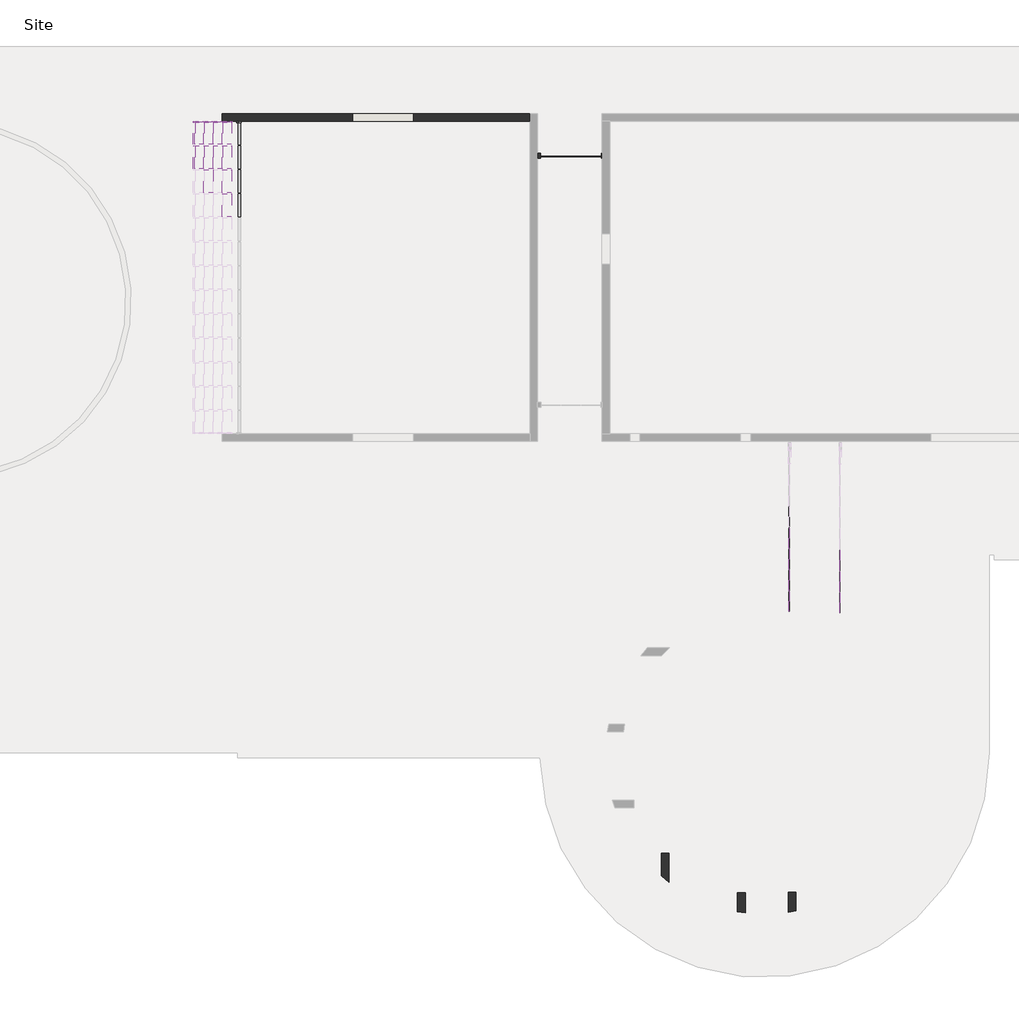
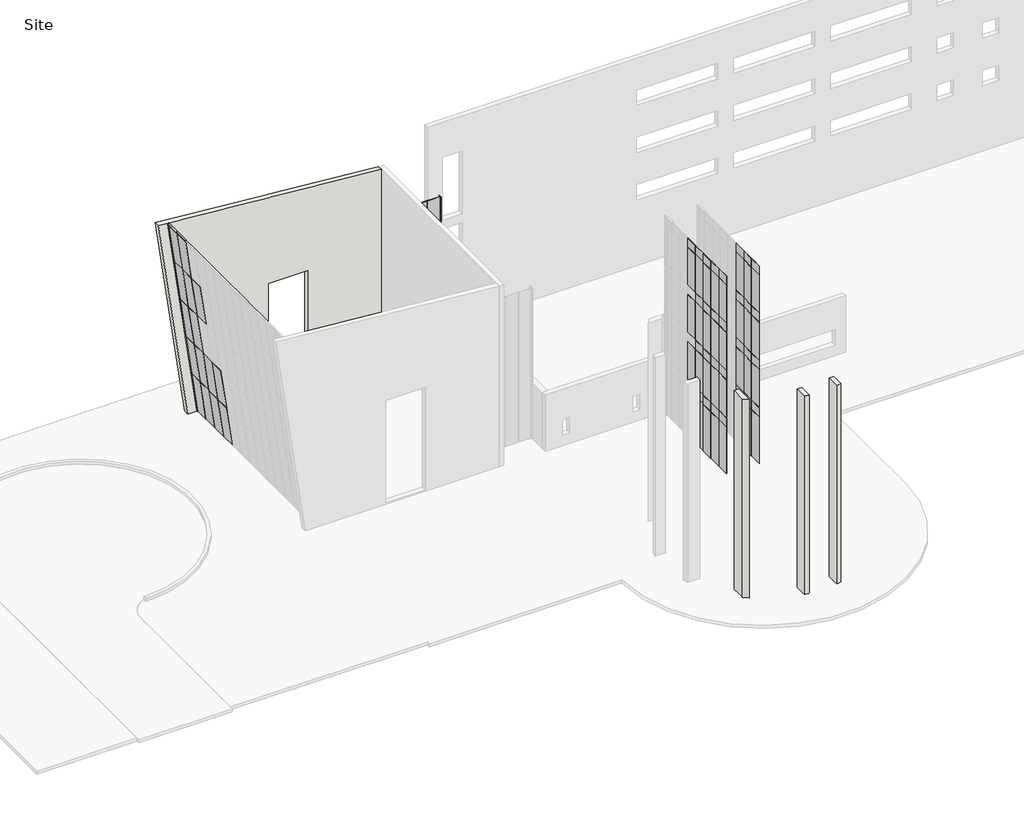
# One storey, part 2 of 4: 79 plates, 7 members, 6 walls.
"""IFC4 building model written with IfcOpenShell, lengths in millimetres."""

import ifcopenshell
import ifcopenshell.guid

model = None  # the IFC model being written
_history = None  # IfcOwnerHistory: only IFC2X3 demands one
_inside = {}  # id of a spatial element -> (the spatial element, [elements in it])
_under = {}  # id of a project, library or spatial element -> (it, [spatial elements below it])
_declared = {}  # id of a project -> (the project, [libraries it declares])
_typed = {}  # id of a type object -> (the type object, [elements of that type])
_made_of = {}  # id of a material, layer set ... -> (it, [elements and type objects made of it])


def new_model(schema):
    """Start an empty IFC model of exactly this schema.

    Asked for "IFC4X3", IfcOpenShell would pick the latest addendum, in which some entities
    have other attributes; the version numbers below select the first issue.
    IFC2X3 requires an IfcOwnerHistory on every rooted entity: one is made here for all.
    """
    global model, _history
    if schema == "IFC4X3":
        model = ifcopenshell.file(schema_version=(4, 3, 0, 0))
    else:
        model = ifcopenshell.file(schema=schema)
    _inside.clear()
    _under.clear()
    _declared.clear()
    _typed.clear()
    _made_of.clear()
    _history = None
    if model.schema == "IFC2X3":
        org = make("IfcOrganization", Name="unknown")
        user = make(
            "IfcPersonAndOrganization",
            ThePerson=make("IfcPerson", FamilyName="unknown"),
            TheOrganization=org,
        )
        app = make(
            "IfcApplication",
            ApplicationDeveloper=org,
            Version="unknown",
            ApplicationFullName="unknown",
            ApplicationIdentifier="unknown",
        )
        _history = make(
            "IfcOwnerHistory",
            OwningUser=user,
            OwningApplication=app,
            ChangeAction="ADDED",
            CreationDate=0,
        )
    return model


def make(cls, **values):
    """One entity of the class cls with the attributes given. An attribute that is None is left unset."""
    return model.create_entity(
        cls, **{name: value for name, value in values.items() if value is not None}
    )


def rooted(cls, **values):
    """An entity with a GlobalId (a new one), such as an element, a storey or a relation."""
    return make(cls, GlobalId=ifcopenshell.guid.new(), OwnerHistory=_history, **values)


def si_unit(unit_type, name, prefix=None):
    """IfcSIUnit, for example si_unit("LENGTHUNIT", "METRE", prefix="MILLI")."""
    return make("IfcSIUnit", UnitType=unit_type, Prefix=prefix, Name=name)


def assignment(units):
    """IfcUnitAssignment: the units of a project."""
    return None if units is None else make("IfcUnitAssignment", Units=units)


def point(xyz):
    """IfcCartesianPoint."""
    return None if xyz is None else make("IfcCartesianPoint", Coordinates=xyz)


def direction(xyz):
    """IfcDirection."""
    return None if xyz is None else make("IfcDirection", DirectionRatios=xyz)


def frame(location, z_axis=None, x_axis=None):
    """IfcAxis2Placement3D, a coordinate frame: its origin and axes. An axis left out is left unset."""
    return make(
        "IfcAxis2Placement3D",
        Location=point(location),
        Axis=direction(z_axis),
        RefDirection=direction(x_axis),
    )


def frame_2d(location, x_axis=None):
    """IfcAxis2Placement2D, a coordinate frame in the plane: its origin and x axis."""
    return make(
        "IfcAxis2Placement2D", Location=point(location), RefDirection=direction(x_axis)
    )


def origin():
    """The frame at (0, 0, 0) with its axes left unset."""
    return frame((0.0, 0.0, 0.0))


def origin_with_axes():
    """The frame at (0, 0, 0) with the z axis (0, 0, 1) and the x axis (1, 0, 0) written out."""
    return frame((0.0, 0.0, 0.0), z_axis=(0.0, 0.0, 1.0), x_axis=(1.0, 0.0, 0.0))


def place(relative_to, where):
    """IfcLocalPlacement: puts the frame where relative to a parent placement (None: the world)."""
    return make(
        "IfcLocalPlacement", PlacementRelTo=relative_to, RelativePlacement=where
    )


def context(
    kind, dimensions, precision=None, world=None, true_north=None, identifier=None
):
    """IfcGeometricRepresentationContext, for example the 3D "Model" context."""
    return make(
        "IfcGeometricRepresentationContext",
        ContextIdentifier=identifier,
        ContextType=kind,
        CoordinateSpaceDimension=dimensions,
        Precision=precision,
        WorldCoordinateSystem=world,
        TrueNorth=true_north,
    )


def project(units=None, contexts=None):
    """IfcProject with its units and contexts."""
    return rooted(
        "IfcProject",
        Name="project",
        RepresentationContexts=contexts,
        UnitsInContext=assignment(units),
    )


def spatial(cls, under=None, at=None, **own):
    """A site, building, storey or space (cls), placed at a placement, below another one or the project."""
    s = rooted(cls, ObjectPlacement=at, **own)
    if under is not None:
        _under.setdefault(under.id(), (under, []))[1].append(s)
    return s


def polyline(points):
    """IfcPolyline through the points."""
    return make("IfcPolyline", Points=[point(p) for p in points])


def circle_curve(where, radius):
    """IfcCircle in the frame where."""
    return make("IfcCircle", Position=where, Radius=radius)


def trimmed(basis, trim1, trim2, sense, master):
    """IfcTrimmedCurve: the piece of a basis curve between two trims."""
    return make(
        "IfcTrimmedCurve",
        BasisCurve=basis,
        Trim1=trim1,
        Trim2=trim2,
        SenseAgreement=sense,
        MasterRepresentation=master,
    )


def segment(curve, same_sense, transition):
    """IfcCompositeCurveSegment."""
    return make(
        "IfcCompositeCurveSegment",
        Transition=transition,
        SameSense=same_sense,
        ParentCurve=curve,
    )


def composite_curve(segments, self_intersect=None):
    """IfcCompositeCurve: segments joined end to end."""
    return make("IfcCompositeCurve", Segments=segments, SelfIntersect=self_intersect)


def outline(outer, holes=None, kind="AREA"):
    """IfcArbitraryClosedProfileDef: a profile drawn as a closed curve; with holes, ...WithVoids."""
    if holes is None:
        return make("IfcArbitraryClosedProfileDef", ProfileType=kind, OuterCurve=outer)
    return make(
        "IfcArbitraryProfileDefWithVoids",
        ProfileType=kind,
        OuterCurve=outer,
        InnerCurves=holes,
    )


def extrude(swept, where, along, depth):
    """IfcExtrudedAreaSolid: the profile swept, set in the frame where, extruded along a direction by depth."""
    return make(
        "IfcExtrudedAreaSolid",
        SweptArea=swept,
        Position=where,
        ExtrudedDirection=direction(along),
        Depth=depth,
    )


def shape(context_of_items, identifier, shape_type, items):
    """IfcShapeRepresentation: the items that make up one representation, for example the "Body"."""
    return make(
        "IfcShapeRepresentation",
        ContextOfItems=context_of_items,
        RepresentationIdentifier=identifier,
        RepresentationType=shape_type,
        Items=items,
    )


def source(mapping_origin, context_of_items, identifier, shape_type, items):
    """IfcRepresentationMap: a shape defined once, which mapped items show again and again."""
    return make(
        "IfcRepresentationMap",
        MappingOrigin=mapping_origin,
        MappedRepresentation=shape(context_of_items, identifier, shape_type, items),
    )


def transform(
    local_origin,
    x_axis=None,
    y_axis=None,
    z_axis=None,
    scale=None,
    scale2=None,
    scale3=None,
    uniform=True,
):
    """IfcCartesianTransformationOperator3D, or its non-uniform kind. x_axis, y_axis, z_axis: its Axis1, 2, 3."""
    if uniform:
        return make(
            "IfcCartesianTransformationOperator3D",
            Axis1=direction(x_axis),
            Axis2=direction(y_axis),
            LocalOrigin=point(local_origin),
            Scale=scale,
            Axis3=direction(z_axis),
        )
    return make(
        "IfcCartesianTransformationOperator3DnonUniform",
        Axis1=direction(x_axis),
        Axis2=direction(y_axis),
        LocalOrigin=point(local_origin),
        Scale=scale,
        Axis3=direction(z_axis),
        Scale2=scale2,
        Scale3=scale3,
    )


def mapped(mapping_source, mapping_target):
    """IfcMappedItem: shows the shape of a source again, moved by a transform."""
    return make(
        "IfcMappedItem", MappingSource=mapping_source, MappingTarget=mapping_target
    )


def made_of(thing, what):
    """Note that an element or type object is made of a material, layer set ...; save() writes the relation."""
    if what is not None:
        _made_of.setdefault(what.id(), (what, []))[1].append(thing)
    return thing


def element(
    cls,
    number,
    at=None,
    inside=None,
    cuts=None,
    type_object=None,
    material=None,
    context=None,
    identifier="Body",
    shape_type=None,
    held_by="IfcProductDefinitionShape",
    body=None,
    shapes=None,
    **own,
):
    """One element of the class cls, such as IfcWall. Its Tag is "e" and its number.

    at: its placement. inside: the storey or other place that contains it. cuts: it is an
    opening in that element (IfcRelVoidsElement). A single representation is given by context,
    identifier, shape_type and body (its items); several are given by shapes. held_by: the class
    of the entity that holds the representations. save() writes the other relations.
    """
    e = rooted(cls, Tag="e%d" % number, ObjectPlacement=at, **own)
    if body is not None:
        shapes = [shape(context, identifier, shape_type, body)]
    if shapes is not None:
        e.Representation = make(held_by, Representations=shapes)
    if inside is not None:
        _inside.setdefault(inside.id(), (inside, []))[1].append(e)
    if cuts is not None:
        rooted(
            "IfcRelVoidsElement", RelatingBuildingElement=cuts, RelatedOpeningElement=e
        )
    if type_object is not None:
        _typed.setdefault(type_object.id(), (type_object, []))[1].append(e)
    return made_of(e, material)


def aggregate(whole, parts):
    """IfcRelAggregates: a whole, such as a stair, and the parts it consists of."""
    return rooted("IfcRelAggregates", RelatingObject=whole, RelatedObjects=parts)


def save(model, path):
    """Write the relations noted so far, then the file.

    IfcRelAggregates (storeys below a building ...), IfcRelContainedInSpatialStructure (elements
    in a storey), IfcRelDefinesByType, IfcRelAssociatesMaterial and IfcRelDeclares: one each for
    every whole, place, type object, material and project.
    """
    for whole, parts in _under.values():
        aggregate(whole, parts)
    for where, things in _inside.values():
        rooted(
            "IfcRelContainedInSpatialStructure",
            RelatedElements=things,
            RelatingStructure=where,
        )
    for kind, things in _typed.values():
        rooted("IfcRelDefinesByType", RelatedObjects=things, RelatingType=kind)
    for what, things in _made_of.values():
        rooted("IfcRelAssociatesMaterial", RelatedObjects=things, RelatingMaterial=what)
    for by, libraries in _declared.values():
        rooted("IfcRelDeclares", RelatingContext=by, RelatedDefinitions=libraries)
    model.write(path)


def member_f8a9089e(model_context):
    return source(origin(), model_context, "Body", "SweptSolid", [
        extrude(outline(polyline([(0.0, 63.5), (0.0, -63.5), (-63.5, -63.5), (-63.5, 63.5), (0.0, 63.5)])), frame((0.0, 0.0, -1320.067308), z_axis=(0.0, 0.0, 1.0), x_axis=(1.0, 0.0, 0.0)), (0.0, 0.0, 1.0), 1320.067308),
    ])


def member_5e02c13a(model_context):
    return source(origin(), model_context, "Body", "SweptSolid", [
        extrude(outline(polyline([(0.0, 63.5), (0.0, -63.5), (-63.5, -63.5), (-63.5, 63.5), (0.0, 63.5)])), frame((0.0, 0.0, -1383.5673076), z_axis=(0.0, 0.0, 1.0), x_axis=(1.0, 0.0, 0.0)), (0.0, 0.0, 1.0), 1383.5673076),
    ])


def member_50cd645d(model_context):
    return source(origin(), model_context, "Body", "SweptSolid", [
        extrude(outline(polyline([(0.0, 63.5), (0.0, -63.5), (-63.5, -63.5), (-63.5, 63.5), (0.0, 63.5)])), frame((0.0, 0.0, -4003.5335741), z_axis=(0.0, 0.0, 1.0), x_axis=(1.0, 0.0, 0.0)), (0.0, 0.0, 1.0), 4003.5335741),
    ])


def member_5d333a65(model_context):
    return source(origin(), model_context, "Body", "SweptSolid", [
        extrude(outline(polyline([(0.0, 63.5), (0.0, -63.5), (-63.5, -63.5), (-63.5, 63.5), (0.0, 63.5)])), frame((0.0, 0.0, -3971.7835741), z_axis=(0.0, 0.0, 1.0), x_axis=(1.0, 0.0, 0.0)), (0.0, 0.0, 1.0), 3971.7835741),
    ])


def system_panel_glazed_908aa4c7(model_context):
    return source(origin(), model_context, "Body", "SweptSolid", [
        extrude(outline(polyline([(593.725, 19.05), (-593.725, 19.05), (-593.725, 44.45), (593.725, 44.45), (593.725, 19.05)])), origin_with_axes(), (0.0, 0.0, 1.0), 4629.15),
    ])


def system_panel_glazed_38880ecf(model_context):
    return source(origin(), model_context, "Body", "SweptSolid", [
        extrude(outline(polyline([(587.8744819, 19.05), (-587.8744819, 19.05), (-587.8744819, 44.45), (587.8744819, 44.45), (587.8744819, 19.05)])), origin_with_axes(), (0.0, 0.0, 1.0), 4629.15),
    ])


def system_panel_glazed_26f8e022(model_context):
    return source(origin(), model_context, "Body", "SweptSolid", [
        extrude(outline(polyline([(603.7494819, 19.05), (-603.7494819, 19.05), (-603.7494819, 44.45), (603.7494819, 44.45), (603.7494819, 19.05)])), origin_with_axes(), (0.0, 0.0, 1.0), 4629.15),
    ])


def system_panel_glazed_31d10065(model_context):
    return source(origin(), model_context, "Body", "SweptSolid", [
        extrude(outline(polyline([(609.6, 19.05), (-609.6, 19.05), (-609.6, 44.45), (609.6, 44.45), (609.6, 19.05)])), origin_with_axes(), (0.0, 0.0, 1.0), 4629.15),
    ])


def system_panel_glazed_d00c2bb3(model_context):
    return source(origin(), model_context, "Body", "SweptSolid", [
        extrude(outline(polyline([(609.5367635, 19.05), (-609.5367635, 19.05), (-609.5367635, 44.45), (609.5367635, 44.45), (609.5367635, 19.05)])), origin_with_axes(), (0.0, 0.0, 1.0), 15087.6),
    ])


def system_panel_glazed_c11227ff(model_context):
    return source(origin(), model_context, "Body", "SweptSolid", [
        extrude(outline(polyline([(593.725, 19.05), (-593.725, 19.05), (-593.725, 44.45), (593.725, 44.45), (593.725, 19.05)])), origin_with_axes(), (0.0, 0.0, 1.0), 3746.5),
    ])


def system_panel_glazed_2b3d2baa(model_context):
    return source(origin(), model_context, "Body", "SweptSolid", [
        extrude(outline(polyline([(609.6, 19.05), (-609.6, 19.05), (-609.6, 44.45), (609.6, 44.45), (609.6, 19.05)])), origin_with_axes(), (0.0, 0.0, 1.0), 3746.5),
    ])


def system_panel_glazed_00a161e3(model_context):
    return source(origin(), model_context, "Body", "SweptSolid", [
        extrude(outline(polyline([(593.725, 19.05), (-593.725, 19.05), (-593.725, 44.45), (593.725, 44.45), (593.725, 19.05)])), origin_with_axes(), (0.0, 0.0, 1.0), 850.9),
    ])


def system_panel_glazed_8fe7ab7d(model_context):
    return source(origin(), model_context, "Body", "SweptSolid", [
        extrude(outline(polyline([(609.6, 19.05), (-609.6, 19.05), (-609.6, 44.45), (609.6, 44.45), (609.6, 19.05)])), origin_with_axes(), (0.0, 0.0, 1.0), 850.9),
    ])


def system_panel_glazed_2ccc015e(model_context):
    return source(origin(), model_context, "Body", "SweptSolid", [
        extrude(outline(polyline([(593.725, 19.05), (-593.725, 19.05), (-593.725, 44.45), (593.725, 44.45), (593.725, 19.05)])), origin_with_axes(), (0.0, 0.0, 1.0), 819.15),
    ])


def system_panel_glazed_636dec6d(model_context):
    return source(origin(), model_context, "Body", "SweptSolid", [
        extrude(outline(polyline([(609.6, 19.05), (-609.6, 19.05), (-609.6, 44.45), (609.6, 44.45), (609.6, 19.05)])), origin_with_axes(), (0.0, 0.0, 1.0), 819.15),
    ])


def system_panel_glazed_4a693619(model_context):
    return source(origin(), model_context, "Body", "SweptSolid", [
        extrude(outline(polyline([(587.8744819, 19.05), (-587.8744819, 19.05), (-587.8744819, 44.45), (587.8744819, 44.45), (587.8744819, 19.05)])), origin_with_axes(), (0.0, 0.0, 1.0), 3746.5),
    ])


def system_panel_glazed_35bb093a(model_context):
    return source(origin(), model_context, "Body", "SweptSolid", [
        extrude(outline(polyline([(603.7494819, 19.05), (-603.7494819, 19.05), (-603.7494819, 44.45), (603.7494819, 44.45), (603.7494819, 19.05)])), origin_with_axes(), (0.0, 0.0, 1.0), 3746.5),
    ])


def system_panel_glazed_f91df05e(model_context):
    return source(origin(), model_context, "Body", "SweptSolid", [
        extrude(outline(polyline([(660.033654, 19.05), (-660.033654, 19.05), (-660.033654, 44.45), (660.033654, 44.45), (660.033654, 19.05)])), origin_with_axes(), (0.0, 0.0, 1.0), 3908.2835741),
    ])


def system_panel_glazed_78b5b18d(model_context):
    return source(origin(), model_context, "Body", "SweptSolid", [
        extrude(outline(polyline([(691.7836538, 19.05), (-691.7836538, 19.05), (-691.7836538, 44.45), (691.7836538, 44.45), (691.7836538, 19.05)])), origin_with_axes(), (0.0, 0.0, 1.0), 3908.2835741),
    ])


def system_panel_metal_panel_ca084d4b(model_context):
    return source(origin(), model_context, "Body", "SweptSolid", [
        extrude(outline(polyline([(587.8744819, 19.05), (-587.8744819, 19.05), (-587.8744819, 44.45), (587.8744819, 44.45), (587.8744819, 19.05)])), origin_with_axes(), (0.0, 0.0, 1.0), 819.15),
    ])


def system_panel_metal_panel_947f48db(model_context):
    return source(origin(), model_context, "Body", "SweptSolid", [
        extrude(outline(polyline([(603.7494819, 19.05), (-603.7494819, 19.05), (-603.7494819, 44.45), (603.7494819, 44.45), (603.7494819, 19.05)])), origin_with_axes(), (0.0, 0.0, 1.0), 819.15),
    ])


def system_panel_metal_panel_f9c2a482(model_context):
    return source(origin(), model_context, "Body", "SweptSolid", [
        extrude(outline(polyline([(587.8744819, 19.05), (-587.8744819, 19.05), (-587.8744819, 44.45), (587.8744819, 44.45), (587.8744819, 19.05)])), origin_with_axes(), (0.0, 0.0, 1.0), 850.9),
    ])


def system_panel_metal_panel_dcd9a435(model_context):
    return source(origin(), model_context, "Body", "SweptSolid", [
        extrude(outline(polyline([(603.7494819, 19.05), (-603.7494819, 19.05), (-603.7494819, 44.45), (603.7494819, 44.45), (603.7494819, 19.05)])), origin_with_axes(), (0.0, 0.0, 1.0), 850.9),
    ])


model = new_model("IFC4")

# Units and contexts
model_context = context("Model", 3, world=origin())
ifc_project = project(units=[si_unit("LENGTHUNIT", "METRE", prefix="MILLI")], contexts=[model_context])

# Site, building, storey
site = spatial("IfcSite", under=ifc_project)
building = spatial("IfcBuilding", under=site)
storey = spatial("IfcBuildingStorey", under=building, Name="Site", Elevation=-152.4)

# Members
placement = place(None, origin())
member_shape = member_f8a9089e(model_context)
element("IfcMember", 1, ObjectType="Rectangular Mullion1 : 2.5\" x 5\" rectangular", at=placement, inside=storey, context=model_context, shape_type="MappedRepresentation", body=[
    mapped(member_shape, transform((-27908.8595656, 55983.1320811, 19574.3667708), x_axis=(-0.13917310096006533, 0.0, 0.9902680687415704), y_axis=(-0.9902680687415704, 0.0, -0.13917310096006533), z_axis=(0.0, -1.0, 0.0))),
])
member_2_shape = member_5e02c13a(model_context)
element("IfcMember", 2, ObjectType="Rectangular Mullion1 : 2.5\" x 5\" rectangular", at=placement, inside=storey, context=model_context, shape_type="MappedRepresentation", body=[
    mapped(member_2_shape, transform((-27908.8595656, 54536.0647734, 19574.3667708), x_axis=(-0.13917310096006533, 0.0, 0.9902680687415704), y_axis=(-0.9902680687415704, 0.0, -0.13917310096006533), z_axis=(0.0, -1.0, 0.0))),
])
member_3_shape = member_50cd645d(model_context)
element("IfcMember", 3, ObjectType="Rectangular Mullion1 : 2.5\" x 5\" rectangular", at=placement, inside=storey, context=model_context, shape_type="MappedRepresentation", body=[
    mapped(member_3_shape, transform((-27908.8595656, 57366.699389, 19574.3667708), x_axis=(0.0, 1.0, 0.0), y_axis=(-0.9902680687415703, 0.0, -0.13917310096006566), z_axis=(-0.13917310096006566, 0.0, 0.9902680687415703))),
])
element("IfcMember", 4, ObjectType="Rectangular Mullion1 : 2.5\" x 5\" rectangular", at=placement, inside=storey, context=model_context, shape_type="MappedRepresentation", body=[
    mapped(member_3_shape, transform((-25693.3790742, 57366.699389, 3810.4039622), x_axis=(0.0, 1.0, 0.0), y_axis=(-0.9902680687415704, 0.0, -0.13917310096006544), z_axis=(-0.1391731009600654, 0.0, 0.9902680687415703))),
])
member_4_shape = member_5d333a65(model_context)
element("IfcMember", 5, ObjectType="Rectangular Mullion1 : 2.5\" x 5\" rectangular", at=placement, inside=storey, context=model_context, shape_type="MappedRepresentation", body=[
    mapped(member_4_shape, transform((-26246.1445106, 57366.699389, 7743.5344115), x_axis=(0.0, 1.0, 0.0), y_axis=(-0.9902680687415703, 0.0, -0.13917310096006563), z_axis=(-0.1391731009600656, 0.0, 0.9902680687415701))),
])
element("IfcMember", 6, ObjectType="Rectangular Mullion1 : 2.5\" x 5\" rectangular", at=placement, inside=storey, context=model_context, shape_type="MappedRepresentation", body=[
    mapped(member_4_shape, transform((-26798.9099469, 57366.699389, 11676.6648609), x_axis=(0.0, 1.0, 0.0), y_axis=(-0.9902680687415704, 0.0, -0.13917310096006574), z_axis=(-0.13917310096006574, 0.0, 0.9902680687415704))),
])
element("IfcMember", 7, ObjectType="Rectangular Mullion1 : 2.5\" x 5\" rectangular", at=placement, inside=storey, context=model_context, shape_type="MappedRepresentation", body=[
    mapped(member_4_shape, transform((-27351.6753833, 57366.699389, 15609.7953102), x_axis=(0.0, 1.0, 0.0), y_axis=(-0.9902680687415705, 0.0, -0.13917310096006458), z_axis=(-0.13917310096006458, 0.0, 0.9902680687415705))),
])

# Plates
system_panel_glazed_shape = system_panel_glazed_908aa4c7(model_context)
element("IfcPlate", 8, ObjectType="System Panel : Glazed", at=placement, inside=storey, context=model_context, shape_type="MappedRepresentation", body=[
    mapped(system_panel_glazed_shape, transform((10878.8276119, 28482.136889, -88.9), x_axis=(0.0, 1.0, 0.0), y_axis=(-1.0, 0.0, 0.0), z_axis=(0.0, 0.0, 1.0))),
])
system_panel_glazed_2_shape = system_panel_glazed_38880ecf(model_context)
element("IfcPlate", 9, ObjectType="System Panel : Glazed", at=placement, inside=storey, context=model_context, shape_type="MappedRepresentation", body=[
    mapped(system_panel_glazed_2_shape, transform((7830.8276119, 28569.8946611, -88.9), x_axis=(0.0, 1.0, 0.0), y_axis=(-1.0, 0.0, 0.0), z_axis=(0.0, 0.0, 1.0))),
])
system_panel_glazed_3_shape = system_panel_glazed_26f8e022(model_context)
element("IfcPlate", 10, ObjectType="System Panel : Glazed", at=placement, inside=storey, context=model_context, shape_type="MappedRepresentation", body=[
    mapped(system_panel_glazed_3_shape, transform((7830.8276119, 33638.015516, -88.9), x_axis=(0.0, 1.0, 0.0), y_axis=(-1.0, 0.0, 0.0), z_axis=(0.0, 0.0, 1.0))),
])
element("IfcPlate", 11, ObjectType="System Panel : Glazed", at=placement, inside=storey, context=model_context, shape_type="MappedRepresentation", body=[
    mapped(system_panel_glazed_3_shape, transform((7830.8276119, 31096.0175885, -88.9), x_axis=(0.0, 1.0, 0.0), y_axis=(-1.0, 0.0, 0.0), z_axis=(0.0, 0.0, 1.0))),
])
element("IfcPlate", 12, ObjectType="System Panel : Glazed", at=placement, inside=storey, context=model_context, shape_type="MappedRepresentation", body=[
    mapped(system_panel_glazed_3_shape, transform((7830.8276119, 32367.0165522, -88.9), x_axis=(0.0, 1.0, 0.0), y_axis=(-1.0, 0.0, 0.0), z_axis=(0.0, 0.0, 1.0))),
])
element("IfcPlate", 13, ObjectType="System Panel : Glazed", at=placement, inside=storey, context=model_context, shape_type="MappedRepresentation", body=[
    mapped(system_panel_glazed_3_shape, transform((7830.8276119, 29825.0186248, -88.9), x_axis=(0.0, 1.0, 0.0), y_axis=(-1.0, 0.0, 0.0), z_axis=(0.0, 0.0, 1.0))),
])
system_panel_glazed_4_shape = system_panel_glazed_31d10065(model_context)
element("IfcPlate", 14, ObjectType="System Panel : Glazed", at=placement, inside=storey, context=model_context, shape_type="MappedRepresentation", body=[
    mapped(system_panel_glazed_4_shape, transform((10878.8276119, 31031.661889, -88.9), x_axis=(0.0, 1.0, 0.0), y_axis=(-1.0, 0.0, 0.0), z_axis=(0.0, 0.0, 1.0))),
])
element("IfcPlate", 15, ObjectType="System Panel : Glazed", at=placement, inside=storey, context=model_context, shape_type="MappedRepresentation", body=[
    mapped(system_panel_glazed_4_shape, transform((10878.8276119, 29748.961889, -88.9), x_axis=(0.0, 1.0, 0.0), y_axis=(-1.0, 0.0, 0.0), z_axis=(0.0, 0.0, 1.0))),
])
system_panel_glazed_5_shape = system_panel_glazed_d00c2bb3(model_context)
element("IfcPlate", 16, ObjectType="System Panel : Glazed", at=placement, inside=storey, context=model_context, shape_type="MappedRepresentation", body=[
    mapped(system_panel_glazed_5_shape, transform((-4081.74698, 55307.711889, -152.4), x_axis=(-1.0, 0.0, 0.0), y_axis=(0.0, -1.0, 0.0), z_axis=(0.0, 0.0, 1.0))),
])
element("IfcPlate", 17, ObjectType="System Panel : Glazed", at=placement, inside=storey, context=model_context, shape_type="MappedRepresentation", body=[
    mapped(system_panel_glazed_5_shape, transform((-6519.8940341, 55307.711889, -152.4), x_axis=(-1.0, 0.0, 0.0), y_axis=(0.0, -1.0, 0.0), z_axis=(0.0, 0.0, 1.0))),
])
element("IfcPlate", 18, ObjectType="System Panel : Glazed", at=placement, inside=storey, context=model_context, shape_type="MappedRepresentation", body=[
    mapped(system_panel_glazed_5_shape, transform((-5300.8205071, 55307.711889, -152.4), x_axis=(-1.0, 0.0, 0.0), y_axis=(0.0, -1.0, 0.0), z_axis=(0.0, 0.0, 1.0))),
])
system_panel_glazed_6_shape = system_panel_glazed_c11227ff(model_context)
element("IfcPlate", 19, ObjectType="System Panel : Glazed", at=placement, inside=storey, context=model_context, shape_type="MappedRepresentation", body=[
    mapped(system_panel_glazed_6_shape, transform((10878.8276119, 28482.136889, 14966.95), x_axis=(0.0, 1.0, 0.0), y_axis=(-1.0, 0.0, 0.0), z_axis=(0.0, 0.0, 1.0))),
])
element("IfcPlate", 20, ObjectType="System Panel : Glazed", at=placement, inside=storey, context=model_context, shape_type="MappedRepresentation", body=[
    mapped(system_panel_glazed_6_shape, transform((10878.8276119, 28482.136889, 10242.55), x_axis=(0.0, 1.0, 0.0), y_axis=(-1.0, 0.0, 0.0), z_axis=(0.0, 0.0, 1.0))),
])
element("IfcPlate", 21, ObjectType="System Panel : Glazed", at=placement, inside=storey, context=model_context, shape_type="MappedRepresentation", body=[
    mapped(system_panel_glazed_6_shape, transform((10878.8276119, 28482.136889, 5518.15), x_axis=(0.0, 1.0, 0.0), y_axis=(-1.0, 0.0, 0.0), z_axis=(0.0, 0.0, 1.0))),
])
system_panel_glazed_7_shape = system_panel_glazed_2b3d2baa(model_context)
element("IfcPlate", 22, ObjectType="System Panel : Glazed", at=placement, inside=storey, context=model_context, shape_type="MappedRepresentation", body=[
    mapped(system_panel_glazed_7_shape, transform((10878.8276119, 29748.961889, 14966.95), x_axis=(0.0, 1.0, 0.0), y_axis=(-1.0, 0.0, 0.0), z_axis=(0.0, 0.0, 1.0))),
])
element("IfcPlate", 23, ObjectType="System Panel : Glazed", at=placement, inside=storey, context=model_context, shape_type="MappedRepresentation", body=[
    mapped(system_panel_glazed_7_shape, transform((10878.8276119, 31031.661889, 14966.95), x_axis=(0.0, 1.0, 0.0), y_axis=(-1.0, 0.0, 0.0), z_axis=(0.0, 0.0, 1.0))),
])
element("IfcPlate", 24, ObjectType="System Panel : Glazed", at=placement, inside=storey, context=model_context, shape_type="MappedRepresentation", body=[
    mapped(system_panel_glazed_7_shape, transform((10878.8276119, 29748.961889, 10242.55), x_axis=(0.0, 1.0, 0.0), y_axis=(-1.0, 0.0, 0.0), z_axis=(0.0, 0.0, 1.0))),
])
element("IfcPlate", 25, ObjectType="System Panel : Glazed", at=placement, inside=storey, context=model_context, shape_type="MappedRepresentation", body=[
    mapped(system_panel_glazed_7_shape, transform((10878.8276119, 31031.661889, 10242.55), x_axis=(0.0, 1.0, 0.0), y_axis=(-1.0, 0.0, 0.0), z_axis=(0.0, 0.0, 1.0))),
])
element("IfcPlate", 26, ObjectType="System Panel : Glazed", at=placement, inside=storey, context=model_context, shape_type="MappedRepresentation", body=[
    mapped(system_panel_glazed_7_shape, transform((10878.8276119, 29748.961889, 5518.15), x_axis=(0.0, 1.0, 0.0), y_axis=(-1.0, 0.0, 0.0), z_axis=(0.0, 0.0, 1.0))),
])
element("IfcPlate", 27, ObjectType="System Panel : Glazed", at=placement, inside=storey, context=model_context, shape_type="MappedRepresentation", body=[
    mapped(system_panel_glazed_7_shape, transform((10878.8276119, 31031.661889, 5518.15), x_axis=(0.0, 1.0, 0.0), y_axis=(-1.0, 0.0, 0.0), z_axis=(0.0, 0.0, 1.0))),
])
system_panel_glazed_8_shape = system_panel_glazed_00a161e3(model_context)
element("IfcPlate", 28, ObjectType="System Panel : Glazed", at=placement, inside=storey, context=model_context, shape_type="MappedRepresentation", body=[
    mapped(system_panel_glazed_8_shape, transform((10878.8276119, 28482.136889, 9328.15), x_axis=(0.0, 1.0, 0.0), y_axis=(-1.0, 0.0, 0.0), z_axis=(0.0, 0.0, 1.0))),
])
element("IfcPlate", 29, ObjectType="System Panel : Glazed", at=placement, inside=storey, context=model_context, shape_type="MappedRepresentation", body=[
    mapped(system_panel_glazed_8_shape, transform((10878.8276119, 28482.136889, 4603.75), x_axis=(0.0, 1.0, 0.0), y_axis=(-1.0, 0.0, 0.0), z_axis=(0.0, 0.0, 1.0))),
])
element("IfcPlate", 30, ObjectType="System Panel : Glazed", at=placement, inside=storey, context=model_context, shape_type="MappedRepresentation", body=[
    mapped(system_panel_glazed_8_shape, transform((10878.8276119, 28482.136889, 14052.55), x_axis=(0.0, 1.0, 0.0), y_axis=(-1.0, 0.0, 0.0), z_axis=(0.0, 0.0, 1.0))),
])
system_panel_glazed_9_shape = system_panel_glazed_8fe7ab7d(model_context)
element("IfcPlate", 31, ObjectType="System Panel : Glazed", at=placement, inside=storey, context=model_context, shape_type="MappedRepresentation", body=[
    mapped(system_panel_glazed_9_shape, transform((10878.8276119, 29748.961889, 9328.15), x_axis=(0.0, 1.0, 0.0), y_axis=(-1.0, 0.0, 0.0), z_axis=(0.0, 0.0, 1.0))),
])
element("IfcPlate", 32, ObjectType="System Panel : Glazed", at=placement, inside=storey, context=model_context, shape_type="MappedRepresentation", body=[
    mapped(system_panel_glazed_9_shape, transform((10878.8276119, 31031.661889, 9328.15), x_axis=(0.0, 1.0, 0.0), y_axis=(-1.0, 0.0, 0.0), z_axis=(0.0, 0.0, 1.0))),
])
element("IfcPlate", 33, ObjectType="System Panel : Glazed", at=placement, inside=storey, context=model_context, shape_type="MappedRepresentation", body=[
    mapped(system_panel_glazed_9_shape, transform((10878.8276119, 29748.961889, 4603.75), x_axis=(0.0, 1.0, 0.0), y_axis=(-1.0, 0.0, 0.0), z_axis=(0.0, 0.0, 1.0))),
])
element("IfcPlate", 34, ObjectType="System Panel : Glazed", at=placement, inside=storey, context=model_context, shape_type="MappedRepresentation", body=[
    mapped(system_panel_glazed_9_shape, transform((10878.8276119, 31031.661889, 4603.75), x_axis=(0.0, 1.0, 0.0), y_axis=(-1.0, 0.0, 0.0), z_axis=(0.0, 0.0, 1.0))),
])
element("IfcPlate", 35, ObjectType="System Panel : Glazed", at=placement, inside=storey, context=model_context, shape_type="MappedRepresentation", body=[
    mapped(system_panel_glazed_9_shape, transform((10878.8276119, 29748.961889, 14052.55), x_axis=(0.0, 1.0, 0.0), y_axis=(-1.0, 0.0, 0.0), z_axis=(0.0, 0.0, 1.0))),
])
element("IfcPlate", 36, ObjectType="System Panel : Glazed", at=placement, inside=storey, context=model_context, shape_type="MappedRepresentation", body=[
    mapped(system_panel_glazed_9_shape, transform((10878.8276119, 31031.661889, 14052.55), x_axis=(0.0, 1.0, 0.0), y_axis=(-1.0, 0.0, 0.0), z_axis=(0.0, 0.0, 1.0))),
])
system_panel_glazed_10_shape = system_panel_glazed_2ccc015e(model_context)
element("IfcPlate", 37, ObjectType="System Panel : Glazed", at=placement, inside=storey, context=model_context, shape_type="MappedRepresentation", body=[
    mapped(system_panel_glazed_10_shape, transform((10878.8276119, 28482.136889, 18776.95), x_axis=(0.0, 1.0, 0.0), y_axis=(-1.0, 0.0, 0.0), z_axis=(0.0, 0.0, 1.0))),
])
system_panel_glazed_11_shape = system_panel_glazed_636dec6d(model_context)
element("IfcPlate", 38, ObjectType="System Panel : Glazed", at=placement, inside=storey, context=model_context, shape_type="MappedRepresentation", body=[
    mapped(system_panel_glazed_11_shape, transform((10878.8276119, 29748.961889, 18776.95), x_axis=(0.0, 1.0, 0.0), y_axis=(-1.0, 0.0, 0.0), z_axis=(0.0, 0.0, 1.0))),
])
element("IfcPlate", 39, ObjectType="System Panel : Glazed", at=placement, inside=storey, context=model_context, shape_type="MappedRepresentation", body=[
    mapped(system_panel_glazed_11_shape, transform((10878.8276119, 31031.661889, 18776.95), x_axis=(0.0, 1.0, 0.0), y_axis=(-1.0, 0.0, 0.0), z_axis=(0.0, 0.0, 1.0))),
])
system_panel_glazed_12_shape = system_panel_glazed_4a693619(model_context)
element("IfcPlate", 40, ObjectType="System Panel : Glazed", at=placement, inside=storey, context=model_context, shape_type="MappedRepresentation", body=[
    mapped(system_panel_glazed_12_shape, transform((7830.8276119, 28569.8946611, 5518.15), x_axis=(0.0, 1.0, 0.0), y_axis=(-1.0, 0.0, 0.0), z_axis=(0.0, 0.0, 1.0))),
])
element("IfcPlate", 41, ObjectType="System Panel : Glazed", at=placement, inside=storey, context=model_context, shape_type="MappedRepresentation", body=[
    mapped(system_panel_glazed_12_shape, transform((7830.8276119, 28569.8946611, 10242.55), x_axis=(0.0, 1.0, 0.0), y_axis=(-1.0, 0.0, 0.0), z_axis=(0.0, 0.0, 1.0))),
])
element("IfcPlate", 42, ObjectType="System Panel : Glazed", at=placement, inside=storey, context=model_context, shape_type="MappedRepresentation", body=[
    mapped(system_panel_glazed_12_shape, transform((7830.8276119, 28569.8946611, 14966.95), x_axis=(0.0, 1.0, 0.0), y_axis=(-1.0, 0.0, 0.0), z_axis=(0.0, 0.0, 1.0))),
])
system_panel_glazed_13_shape = system_panel_glazed_35bb093a(model_context)
element("IfcPlate", 43, ObjectType="System Panel : Glazed", at=placement, inside=storey, context=model_context, shape_type="MappedRepresentation", body=[
    mapped(system_panel_glazed_13_shape, transform((7830.8276119, 29825.0186248, 5518.15), x_axis=(0.0, 1.0, 0.0), y_axis=(-1.0, 0.0, 0.0), z_axis=(0.0, 0.0, 1.0))),
])
element("IfcPlate", 44, ObjectType="System Panel : Glazed", at=placement, inside=storey, context=model_context, shape_type="MappedRepresentation", body=[
    mapped(system_panel_glazed_13_shape, transform((7830.8276119, 31096.0175885, 5518.15), x_axis=(0.0, 1.0, 0.0), y_axis=(-1.0, 0.0, 0.0), z_axis=(0.0, 0.0, 1.0))),
])
element("IfcPlate", 45, ObjectType="System Panel : Glazed", at=placement, inside=storey, context=model_context, shape_type="MappedRepresentation", body=[
    mapped(system_panel_glazed_13_shape, transform((7830.8276119, 32367.0165522, 5518.15), x_axis=(0.0, 1.0, 0.0), y_axis=(-1.0, 0.0, 0.0), z_axis=(0.0, 0.0, 1.0))),
])
element("IfcPlate", 46, ObjectType="System Panel : Glazed", at=placement, inside=storey, context=model_context, shape_type="MappedRepresentation", body=[
    mapped(system_panel_glazed_13_shape, transform((7830.8276119, 33638.015516, 5518.15), x_axis=(0.0, 1.0, 0.0), y_axis=(-1.0, 0.0, 0.0), z_axis=(0.0, 0.0, 1.0))),
])
element("IfcPlate", 47, ObjectType="System Panel : Glazed", at=placement, inside=storey, context=model_context, shape_type="MappedRepresentation", body=[
    mapped(system_panel_glazed_13_shape, transform((7830.8276119, 29825.0186248, 10242.55), x_axis=(0.0, 1.0, 0.0), y_axis=(-1.0, 0.0, 0.0), z_axis=(0.0, 0.0, 1.0))),
])
element("IfcPlate", 48, ObjectType="System Panel : Glazed", at=placement, inside=storey, context=model_context, shape_type="MappedRepresentation", body=[
    mapped(system_panel_glazed_13_shape, transform((7830.8276119, 31096.0175885, 10242.55), x_axis=(0.0, 1.0, 0.0), y_axis=(-1.0, 0.0, 0.0), z_axis=(0.0, 0.0, 1.0))),
])
element("IfcPlate", 49, ObjectType="System Panel : Glazed", at=placement, inside=storey, context=model_context, shape_type="MappedRepresentation", body=[
    mapped(system_panel_glazed_13_shape, transform((7830.8276119, 32367.0165522, 10242.55), x_axis=(0.0, 1.0, 0.0), y_axis=(-1.0, 0.0, 0.0), z_axis=(0.0, 0.0, 1.0))),
])
element("IfcPlate", 50, ObjectType="System Panel : Glazed", at=placement, inside=storey, context=model_context, shape_type="MappedRepresentation", body=[
    mapped(system_panel_glazed_13_shape, transform((7830.8276119, 33638.015516, 10242.55), x_axis=(0.0, 1.0, 0.0), y_axis=(-1.0, 0.0, 0.0), z_axis=(0.0, 0.0, 1.0))),
])
element("IfcPlate", 51, ObjectType="System Panel : Glazed", at=placement, inside=storey, context=model_context, shape_type="MappedRepresentation", body=[
    mapped(system_panel_glazed_13_shape, transform((7830.8276119, 29825.0186248, 14966.95), x_axis=(0.0, 1.0, 0.0), y_axis=(-1.0, 0.0, 0.0), z_axis=(0.0, 0.0, 1.0))),
])
element("IfcPlate", 52, ObjectType="System Panel : Glazed", at=placement, inside=storey, context=model_context, shape_type="MappedRepresentation", body=[
    mapped(system_panel_glazed_13_shape, transform((7830.8276119, 31096.0175885, 14966.95), x_axis=(0.0, 1.0, 0.0), y_axis=(-1.0, 0.0, 0.0), z_axis=(0.0, 0.0, 1.0))),
])
element("IfcPlate", 53, ObjectType="System Panel : Glazed", at=placement, inside=storey, context=model_context, shape_type="MappedRepresentation", body=[
    mapped(system_panel_glazed_13_shape, transform((7830.8276119, 32367.0165522, 14966.95), x_axis=(0.0, 1.0, 0.0), y_axis=(-1.0, 0.0, 0.0), z_axis=(0.0, 0.0, 1.0))),
])
element("IfcPlate", 54, ObjectType="System Panel : Glazed", at=placement, inside=storey, context=model_context, shape_type="MappedRepresentation", body=[
    mapped(system_panel_glazed_13_shape, transform((7830.8276119, 33638.015516, 14966.95), x_axis=(0.0, 1.0, 0.0), y_axis=(-1.0, 0.0, 0.0), z_axis=(0.0, 0.0, 1.0))),
])
system_panel_glazed_14_shape = system_panel_glazed_f91df05e(model_context)
element("IfcPlate", 55, ObjectType="System Panel : Glazed", at=placement, inside=storey, context=model_context, shape_type="MappedRepresentation", body=[
    mapped(system_panel_glazed_14_shape, transform((-25145.0323838, 56643.165735, -91.285476), x_axis=(0.0, -1.0, 0.0), y_axis=(0.9902680687415704, 0.0, 0.13917310096006547), z_axis=(-0.13917310096006547, 0.0, 0.9902680687415704))),
])
element("IfcPlate", 56, ObjectType="System Panel : Glazed", at=placement, inside=storey, context=model_context, shape_type="MappedRepresentation", body=[
    mapped(system_panel_glazed_14_shape, transform((-25697.7978202, 56643.165735, 3841.8449733), x_axis=(0.0, -1.0, 0.0), y_axis=(0.9902680687415704, 0.0, 0.13917310096006533), z_axis=(-0.13917310096006533, 0.0, 0.9902680687415704))),
])
element("IfcPlate", 57, ObjectType="System Panel : Glazed", at=placement, inside=storey, context=model_context, shape_type="MappedRepresentation", body=[
    mapped(system_panel_glazed_14_shape, transform((-26250.5632565, 56643.165735, 7774.9754227), x_axis=(0.0, -1.0, 0.0), y_axis=(0.9902680687415704, 0.0, 0.13917310096006533), z_axis=(-0.13917310096006533, 0.0, 0.9902680687415704))),
])
element("IfcPlate", 58, ObjectType="System Panel : Glazed", at=placement, inside=storey, context=model_context, shape_type="MappedRepresentation", body=[
    mapped(system_panel_glazed_14_shape, transform((-26803.3286929, 56643.165735, 11708.105872), x_axis=(0.0, -1.0, 0.0), y_axis=(0.9902680687415704, 0.0, 0.13917310096006533), z_axis=(-0.13917310096006533, 0.0, 0.9902680687415704))),
])
element("IfcPlate", 59, ObjectType="System Panel : Glazed", at=placement, inside=storey, context=model_context, shape_type="MappedRepresentation", body=[
    mapped(system_panel_glazed_14_shape, transform((-27356.0941292, 56643.165735, 15641.2363214), x_axis=(0.0, -1.0, 0.0), y_axis=(0.9902680687415704, 0.0, 0.13917310096006533), z_axis=(-0.13917310096006533, 0.0, 0.9902680687415704))),
])
system_panel_glazed_15_shape = system_panel_glazed_78b5b18d(model_context)
element("IfcPlate", 60, ObjectType="System Panel : Glazed", at=placement, inside=storey, context=model_context, shape_type="MappedRepresentation", body=[
    mapped(system_panel_glazed_15_shape, transform((-25145.0323838, 55227.8484272, -91.285476), x_axis=(0.0, -1.0, 0.0), y_axis=(0.9902680687415704, 0.0, 0.13917310096006547), z_axis=(-0.13917310096006547, 0.0, 0.9902680687415704))),
])
element("IfcPlate", 61, ObjectType="System Panel : Glazed", at=placement, inside=storey, context=model_context, shape_type="MappedRepresentation", body=[
    mapped(system_panel_glazed_15_shape, transform((-25145.0323838, 53780.7811196, -91.285476), x_axis=(0.0, -1.0, 0.0), y_axis=(0.9902680687415704, 0.0, 0.13917310096006547), z_axis=(-0.13917310096006547, 0.0, 0.9902680687415704))),
])
element("IfcPlate", 62, ObjectType="System Panel : Glazed", at=placement, inside=storey, context=model_context, shape_type="MappedRepresentation", body=[
    mapped(system_panel_glazed_15_shape, transform((-25145.0323838, 52333.7138119, -91.285476), x_axis=(0.0, -1.0, 0.0), y_axis=(0.9902680687415704, 0.0, 0.13917310096006547), z_axis=(-0.13917310096006547, 0.0, 0.9902680687415704))),
])
element("IfcPlate", 63, ObjectType="System Panel : Glazed", at=placement, inside=storey, context=model_context, shape_type="MappedRepresentation", body=[
    mapped(system_panel_glazed_15_shape, transform((-25697.7978202, 55227.8484272, 3841.8449733), x_axis=(0.0, -1.0, 0.0), y_axis=(0.9902680687415704, 0.0, 0.13917310096006533), z_axis=(-0.13917310096006533, 0.0, 0.9902680687415704))),
])
element("IfcPlate", 64, ObjectType="System Panel : Glazed", at=placement, inside=storey, context=model_context, shape_type="MappedRepresentation", body=[
    mapped(system_panel_glazed_15_shape, transform((-25697.7978202, 53780.7811196, 3841.8449733), x_axis=(0.0, -1.0, 0.0), y_axis=(0.9902680687415704, 0.0, 0.13917310096006533), z_axis=(-0.13917310096006533, 0.0, 0.9902680687415704))),
])
element("IfcPlate", 65, ObjectType="System Panel : Glazed", at=placement, inside=storey, context=model_context, shape_type="MappedRepresentation", body=[
    mapped(system_panel_glazed_15_shape, transform((-25697.7978202, 52333.7138119, 3841.8449733), x_axis=(0.0, -1.0, 0.0), y_axis=(0.9902680687415704, 0.0, 0.13917310096006533), z_axis=(-0.13917310096006533, 0.0, 0.9902680687415704))),
])
element("IfcPlate", 66, ObjectType="System Panel : Glazed", at=placement, inside=storey, context=model_context, shape_type="MappedRepresentation", body=[
    mapped(system_panel_glazed_15_shape, transform((-26250.5632565, 55227.8484272, 7774.9754227), x_axis=(0.0, -1.0, 0.0), y_axis=(0.9902680687415704, 0.0, 0.13917310096006533), z_axis=(-0.13917310096006533, 0.0, 0.9902680687415704))),
])
element("IfcPlate", 67, ObjectType="System Panel : Glazed", at=placement, inside=storey, context=model_context, shape_type="MappedRepresentation", body=[
    mapped(system_panel_glazed_15_shape, transform((-26803.3286929, 55227.8484272, 11708.105872), x_axis=(0.0, -1.0, 0.0), y_axis=(0.9902680687415704, 0.0, 0.13917310096006533), z_axis=(-0.13917310096006533, 0.0, 0.9902680687415704))),
])
element("IfcPlate", 68, ObjectType="System Panel : Glazed", at=placement, inside=storey, context=model_context, shape_type="MappedRepresentation", body=[
    mapped(system_panel_glazed_15_shape, transform((-26803.3286929, 53780.7811196, 11708.105872), x_axis=(0.0, -1.0, 0.0), y_axis=(0.9902680687415704, 0.0, 0.13917310096006533), z_axis=(-0.13917310096006533, 0.0, 0.9902680687415704))),
])
element("IfcPlate", 69, ObjectType="System Panel : Glazed", at=placement, inside=storey, context=model_context, shape_type="MappedRepresentation", body=[
    mapped(system_panel_glazed_15_shape, transform((-27356.0941292, 55227.8484272, 15641.2363214), x_axis=(0.0, -1.0, 0.0), y_axis=(0.9902680687415704, 0.0, 0.13917310096006533), z_axis=(-0.13917310096006533, 0.0, 0.9902680687415704))),
])
system_panel_metal_panel_shape = system_panel_metal_panel_ca084d4b(model_context)
element("IfcPlate", 70, ObjectType="System Panel : Metal Panel", at=placement, inside=storey, context=model_context, shape_type="MappedRepresentation", body=[
    mapped(system_panel_metal_panel_shape, transform((7830.8276119, 28569.8946611, 18776.95), x_axis=(0.0, 1.0, 0.0), y_axis=(-1.0, 0.0, 0.0), z_axis=(0.0, 0.0, 1.0))),
])
system_panel_metal_panel_2_shape = system_panel_metal_panel_947f48db(model_context)
element("IfcPlate", 71, ObjectType="System Panel : Metal Panel", at=placement, inside=storey, context=model_context, shape_type="MappedRepresentation", body=[
    mapped(system_panel_metal_panel_2_shape, transform((7830.8276119, 29825.0186248, 18776.95), x_axis=(0.0, 1.0, 0.0), y_axis=(-1.0, 0.0, 0.0), z_axis=(0.0, 0.0, 1.0))),
])
element("IfcPlate", 72, ObjectType="System Panel : Metal Panel", at=placement, inside=storey, context=model_context, shape_type="MappedRepresentation", body=[
    mapped(system_panel_metal_panel_2_shape, transform((7830.8276119, 31096.0175885, 18776.95), x_axis=(0.0, 1.0, 0.0), y_axis=(-1.0, 0.0, 0.0), z_axis=(0.0, 0.0, 1.0))),
])
element("IfcPlate", 73, ObjectType="System Panel : Metal Panel", at=placement, inside=storey, context=model_context, shape_type="MappedRepresentation", body=[
    mapped(system_panel_metal_panel_2_shape, transform((7830.8276119, 32367.0165522, 18776.95), x_axis=(0.0, 1.0, 0.0), y_axis=(-1.0, 0.0, 0.0), z_axis=(0.0, 0.0, 1.0))),
])
element("IfcPlate", 74, ObjectType="System Panel : Metal Panel", at=placement, inside=storey, context=model_context, shape_type="MappedRepresentation", body=[
    mapped(system_panel_metal_panel_2_shape, transform((7830.8276119, 33638.015516, 18776.95), x_axis=(0.0, 1.0, 0.0), y_axis=(-1.0, 0.0, 0.0), z_axis=(0.0, 0.0, 1.0))),
])
system_panel_metal_panel_3_shape = system_panel_metal_panel_f9c2a482(model_context)
element("IfcPlate", 75, ObjectType="System Panel : Metal Panel", at=placement, inside=storey, context=model_context, shape_type="MappedRepresentation", body=[
    mapped(system_panel_metal_panel_3_shape, transform((7830.8276119, 28569.8946611, 14052.55), x_axis=(0.0, 1.0, 0.0), y_axis=(-1.0, 0.0, 0.0), z_axis=(0.0, 0.0, 1.0))),
])
element("IfcPlate", 76, ObjectType="System Panel : Metal Panel", at=placement, inside=storey, context=model_context, shape_type="MappedRepresentation", body=[
    mapped(system_panel_metal_panel_3_shape, transform((7830.8276119, 28569.8946611, 9328.15), x_axis=(0.0, 1.0, 0.0), y_axis=(-1.0, 0.0, 0.0), z_axis=(0.0, 0.0, 1.0))),
])
element("IfcPlate", 77, ObjectType="System Panel : Metal Panel", at=placement, inside=storey, context=model_context, shape_type="MappedRepresentation", body=[
    mapped(system_panel_metal_panel_3_shape, transform((7830.8276119, 28569.8946611, 4603.75), x_axis=(0.0, 1.0, 0.0), y_axis=(-1.0, 0.0, 0.0), z_axis=(0.0, 0.0, 1.0))),
])
system_panel_metal_panel_4_shape = system_panel_metal_panel_dcd9a435(model_context)
element("IfcPlate", 78, ObjectType="System Panel : Metal Panel", at=placement, inside=storey, context=model_context, shape_type="MappedRepresentation", body=[
    mapped(system_panel_metal_panel_4_shape, transform((7830.8276119, 29825.0186248, 14052.55), x_axis=(0.0, 1.0, 0.0), y_axis=(-1.0, 0.0, 0.0), z_axis=(0.0, 0.0, 1.0))),
])
element("IfcPlate", 79, ObjectType="System Panel : Metal Panel", at=placement, inside=storey, context=model_context, shape_type="MappedRepresentation", body=[
    mapped(system_panel_metal_panel_4_shape, transform((7830.8276119, 31096.0175885, 14052.55), x_axis=(0.0, 1.0, 0.0), y_axis=(-1.0, 0.0, 0.0), z_axis=(0.0, 0.0, 1.0))),
])
element("IfcPlate", 80, ObjectType="System Panel : Metal Panel", at=placement, inside=storey, context=model_context, shape_type="MappedRepresentation", body=[
    mapped(system_panel_metal_panel_4_shape, transform((7830.8276119, 32367.0165522, 14052.55), x_axis=(0.0, 1.0, 0.0), y_axis=(-1.0, 0.0, 0.0), z_axis=(0.0, 0.0, 1.0))),
])
element("IfcPlate", 81, ObjectType="System Panel : Metal Panel", at=placement, inside=storey, context=model_context, shape_type="MappedRepresentation", body=[
    mapped(system_panel_metal_panel_4_shape, transform((7830.8276119, 29825.0186248, 9328.15), x_axis=(0.0, 1.0, 0.0), y_axis=(-1.0, 0.0, 0.0), z_axis=(0.0, 0.0, 1.0))),
])
element("IfcPlate", 82, ObjectType="System Panel : Metal Panel", at=placement, inside=storey, context=model_context, shape_type="MappedRepresentation", body=[
    mapped(system_panel_metal_panel_4_shape, transform((7830.8276119, 31096.0175885, 9328.15), x_axis=(0.0, 1.0, 0.0), y_axis=(-1.0, 0.0, 0.0), z_axis=(0.0, 0.0, 1.0))),
])
element("IfcPlate", 83, ObjectType="System Panel : Metal Panel", at=placement, inside=storey, context=model_context, shape_type="MappedRepresentation", body=[
    mapped(system_panel_metal_panel_4_shape, transform((7830.8276119, 32367.0165522, 9328.15), x_axis=(0.0, 1.0, 0.0), y_axis=(-1.0, 0.0, 0.0), z_axis=(0.0, 0.0, 1.0))),
])
element("IfcPlate", 84, ObjectType="System Panel : Metal Panel", at=placement, inside=storey, context=model_context, shape_type="MappedRepresentation", body=[
    mapped(system_panel_metal_panel_4_shape, transform((7830.8276119, 29825.0186248, 4603.75), x_axis=(0.0, 1.0, 0.0), y_axis=(-1.0, 0.0, 0.0), z_axis=(0.0, 0.0, 1.0))),
])
element("IfcPlate", 85, ObjectType="System Panel : Metal Panel", at=placement, inside=storey, context=model_context, shape_type="MappedRepresentation", body=[
    mapped(system_panel_metal_panel_4_shape, transform((7830.8276119, 31096.0175885, 4603.75), x_axis=(0.0, 1.0, 0.0), y_axis=(-1.0, 0.0, 0.0), z_axis=(0.0, 0.0, 1.0))),
])
element("IfcPlate", 86, ObjectType="System Panel : Metal Panel", at=placement, inside=storey, context=model_context, shape_type="MappedRepresentation", body=[
    mapped(system_panel_metal_panel_4_shape, transform((7830.8276119, 32367.0165522, 4603.75), x_axis=(0.0, 1.0, 0.0), y_axis=(-1.0, 0.0, 0.0), z_axis=(0.0, 0.0, 1.0))),
])

# Walls
element("IfcWall", 87, ObjectType="Stone on CMU", at=placement, inside=storey, context=model_context, shape_type="SweptSolid", body=[
    extrude(outline(composite_curve([segment(polyline([(140.6953567, 12095.1176395), (140.6953567, 13452.4789718), (594.7203567, 13452.4789718), (594.7203567, 11730.5482318)]), True, "CONTINUOUS"), segment(trimmed(circle_curve(frame_2d((6332.5692024, 19341.311889)), 9531.35), [point((594.7203567, 11730.5482318))], [point((140.6953567, 12095.1176395))], False, "CARTESIAN"), True, "CONTINUOUS")], self_intersect=False)), frame((0.0, 0.0, -152.4), z_axis=(0.0, 0.0, 1.0), x_axis=(1.0, 0.0, 0.0)), (0.0, 0.0, 1.0), 19812.0),
])
element("IfcWall", 88, ObjectType="Stone on CMU", at=placement, inside=storey, context=model_context, shape_type="SweptSolid", body=[
    extrude(outline(composite_curve([segment(polyline([(4712.6953567, 9948.6210314), (4712.6953567, 11075.8499375), (5166.7203567, 11075.8499375), (5166.7203567, 9881.5323307)]), True, "CONTINUOUS"), segment(trimmed(circle_curve(frame_2d((6332.5692024, 19341.311889)), 9531.35), [point((5166.7203567, 9881.5323307))], [point((4712.6953567, 9948.6210314))], False, "CARTESIAN"), True, "CONTINUOUS")], self_intersect=False)), frame((0.0, 0.0, -152.4), z_axis=(0.0, 0.0, 1.0), x_axis=(1.0, 0.0, 0.0)), (0.0, 0.0, 1.0), 19812.0),
])
element("IfcWall", 89, ObjectType="Stone on CMU", at=placement, inside=storey, context=model_context, shape_type="SweptSolid", body=[
    extrude(outline(composite_curve([segment(polyline([(7760.6953567, 9917.5605919), (7760.6953567, 11124.3513783), (8214.7203567, 11124.3513783), (8214.7203567, 9997.6434523)]), True, "CONTINUOUS"), segment(trimmed(circle_curve(frame_2d((6332.5692024, 19341.311889)), 9531.35), [point((8214.7203567, 9997.6434523))], [point((7760.6953567, 9917.5605919))], False, "CARTESIAN"), True, "CONTINUOUS")], self_intersect=False)), frame((0.0, 0.0, -152.4), z_axis=(0.0, 0.0, 1.0), x_axis=(1.0, 0.0, 0.0)), (0.0, 0.0, 1.0), 19812.0),
])
element("IfcWall", 90, ObjectType="Stone on CMU", at=placement, inside=storey, context=model_context, shape_type="SweptSolid", body=[
    extrude(outline(polyline([(-152.4, -26050.8432976), (-152.4, -7761.2557976), (17898.2153222, -7761.2557976), (19654.3186785, -28834.4960734), (-152.4, -26050.8432976)]), holes=[polyline([(10210.8, -14747.8432976), (0.0, -14747.8432976), (0.0, -18405.4432976), (10210.8, -18405.4432976), (10210.8, -14747.8432976)])]), frame((0.0, 57366.699389, 0.0), z_axis=(0.0, 1.0, 0.0), x_axis=(0.0, 0.0, 1.0)), (0.0, 0.0, 1.0), 454.025),
])
element("IfcWall", 91, ObjectType="a_Mtl panel on Mtl stud", at=placement, inside=storey, context=model_context, shape_type="SweptSolid", body=[
    extrude(outline(polyline([(-3472.2102165, 55463.286889), (-3419.8227165, 55463.286889), (-3419.8227165, 55152.136889), (-3472.2102165, 55152.136889), (-3472.2102165, 55463.286889)])), frame((0.0, 0.0, -152.4), z_axis=(0.0, 0.0, 1.0), x_axis=(1.0, 0.0, 0.0)), (0.0, 0.0, 1.0), 15087.6),
])
element("IfcWall", 92, ObjectType="a_Mtl panel on Mtl stud", at=placement, inside=storey, context=model_context, shape_type="SweptSolid", body=[
    extrude(outline(polyline([(-7307.2307976, 55463.286889), (-7129.4307976, 55463.286889), (-7129.4307976, 55152.136889), (-7307.2307976, 55152.136889), (-7307.2307976, 55463.286889)])), frame((0.0, 0.0, -152.4), z_axis=(0.0, 0.0, 1.0), x_axis=(1.0, 0.0, 0.0)), (0.0, 0.0, 1.0), 15087.6),
])

save(model, "model.ifc")

# Revit data of these elements
# Type "Rectangular Mullion1 : 2.5\" x 5\" rectangular"
#   built-in parameter 1007304 = 0.416667 (stored number, unit not read)
#   built-in parameter 1007301 = 0.104167 (stored number, unit not read)
#   built-in parameter 1007300 = 0.104167 (stored number, unit not read)
# Type "System Panel : Glazed"
#   Construction Type Id = "GSP4R"
#   Analytic Construction = "1/8 in Pilkington single glazing"
#   Visual Light Transmittance = 0.9
#   Solar Heat Gain Coefficient = 0.86
#   Heat Transfer Coefficient (U) = 1.18115 BTU/(h·ft²·°F)
#   Define Thermal Properties by = 1
# Type "Stone on CMU"
#   Layers, outside or top first: 0' - 2" "Panel Granite 72x48" (function 4); 0' - 3" "Misc. Air Layers - Air Space" (function 3); 0' - 3" "Insulation / Thermal Barriers - Batt insulation" (function 3); 0' - 0" "Vapor / Moisture Barriers - Vapor Retarder" (function 100); 0' - 7 5/8" "Masonry - Concrete Masonry Units" (function 1); 0' - 1 5/8" "Metal - Furring" (function 2); 0' - 0 5/8" "Gypsum Wall Board" (function 5)
# Type "a_Mtl panel on Mtl stud"
#   Layers, outside or top first: 0' - 2" "Metal - Panel" (function 0); 0' - 3" "Misc. Air Layers - Air Space" (function 0); 0' - 0" "Air Barrier - Air Infiltration Barrier" (function 0); 0' - 0 3/4" "Wood - Sheathing - plywood" (function 0); 0' - 6" "Metal - Stud Layer" (function 0); 0' - 0" "Vapor / Moisture Barriers - Vapor Retarder" (function 0); 0' - 0 1/2" no material (function 0)
# Elements 1, 2, 3, 4, 5, 6, 7 (IfcMember, "Rectangular Mullion1 : 2.5\" x 5\" rectangular")
#   Phase Created = New Construction
#   Materials on its faces: "support-frame"
# Elements 8, 9, 10, 11, 12, 13, 14, 15, 16, 17, 18, 19, 20, 21, 22, 23, 24, 25, 26, 27, 28, 29, 30, 31, 32, 33, 34, 35, 36, 37, 38, 39, 40, 41, 42, 43, 44, 45, 46, 47, 48, 49, 50, 51, 52, 53, 54, 55, 56, 57, 58, 59, 60, 61, 62, 63, 64, 65, 66, 67, 68, 69 (IfcPlate, "System Panel : Glazed")
#   Phase Created = New Construction
#   Materials on its faces: "Glass"
# Elements 70, 71, 72, 73, 74, 75, 76, 77, 78, 79, 80, 81, 82, 83, 84, 85, 86 (IfcPlate, "System Panel : Metal Panel")
#   Phase Created = New Construction
#   Materials on its faces: "Aluminum"
# Elements 87, 88, 89 (IfcWall, "Stone on CMU")
#   Top Offset = 0' - 0"
#   Base Offset = 0' - 0"
#   wall height = 65' - 0"
#   Phase Created = New Construction
#   Base Constraint = Site
#   Top Constraint = Roof
#   Materials on its faces: "Default Wall", "Gypsum Wall Board", "Panel Granite 72x48"
# Element 90 (IfcWall, "Stone on CMU")
#   Top Offset = 0' - 0"
#   Base Offset = 0' - 0"
#   wall height = 68' - 0"
#   Phase Created = New Construction
#   Base Constraint = Site
#   Top Constraint = Parapet
#   Materials on its faces: "Default Wall", "Panel Granite 72x48", "Gypsum Wall Board"
# Elements 91, 92 (IfcWall, "a_Mtl panel on Mtl stud")
#   Top Offset = 0' - 0"
#   Base Offset = 0' - 0"
#   wall height = 49' - 6"
#   Phase Created = New Construction
#   Base Constraint = Site
#   Top Constraint = Floor 4
#   Materials on its faces: "Default Wall", "Metal - Panel"
# Materials
#   "Panel Granite 72x48": class "Stone", colour RGB 226 230 231, transparency 0, Cost = 0
#   "Misc. Air Layers - Air Space": class "Miscellaneous", colour RGB 255 255 255, transparency 0
#   "Insulation / Thermal Barriers - Batt insulation": class "Unassigned", colour RGB 127 127 127, transparency 0, Comments = "Rendering appearance not upgraded ", Cost = 0
#   "Vapor / Moisture Barriers - Vapor Retarder": class "Miscellaneous", colour RGB 127 127 127, transparency 0
#   "Masonry - Concrete Masonry Units": class "Concrete", colour RGB 227 227 227, transparency 0
#   "Metal - Furring": class "Metal", colour RGB 199 199 199, transparency 0
#   "Gypsum Wall Board": class "Generic", colour RGB 127 127 127, transparency 0, Description = "Gypsum Wall Board", Cost = 0
#   "Metal - Panel": class "Unassigned", colour RGB 127 127 127, transparency 0
#   "Air Barrier - Air Infiltration Barrier": class "Miscellaneous", colour RGB 127 127 127, transparency 0
#   "Wood - Sheathing - plywood": class "Wood", colour RGB 212 179 113, transparency 0
#   "Metal - Stud Layer": class "Metal", colour RGB 199 199 199, transparency 0
#   "support-frame": class "Unassigned", colour RGB 233 233 233, transparency 0, Cost = 0
#   "Glass": class "Glass", colour RGB 0 128 192, transparency 0.75, Description = "Soda Lime Glass", Cost = 0
#   "Aluminum": class "Metal", colour RGB 247 247 247, transparency 0, Description = "Aluminum 6061", Cost = 0
#   "Default Wall": class "Miscellaneous", colour RGB 128 128 128, transparency 0, Cost = 0
